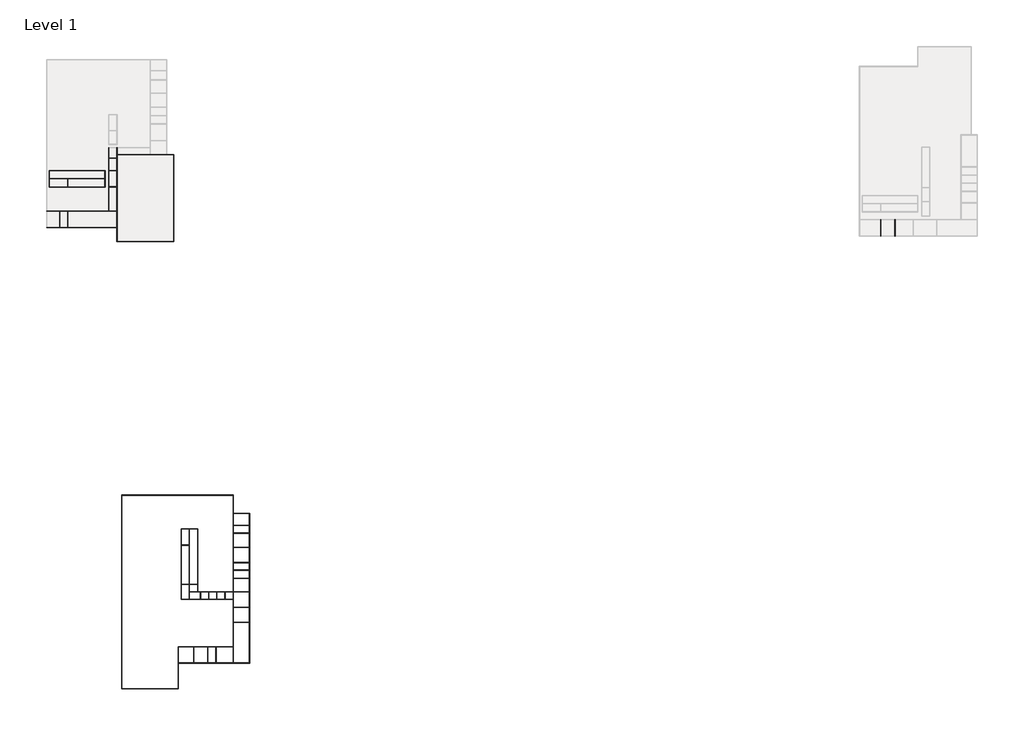
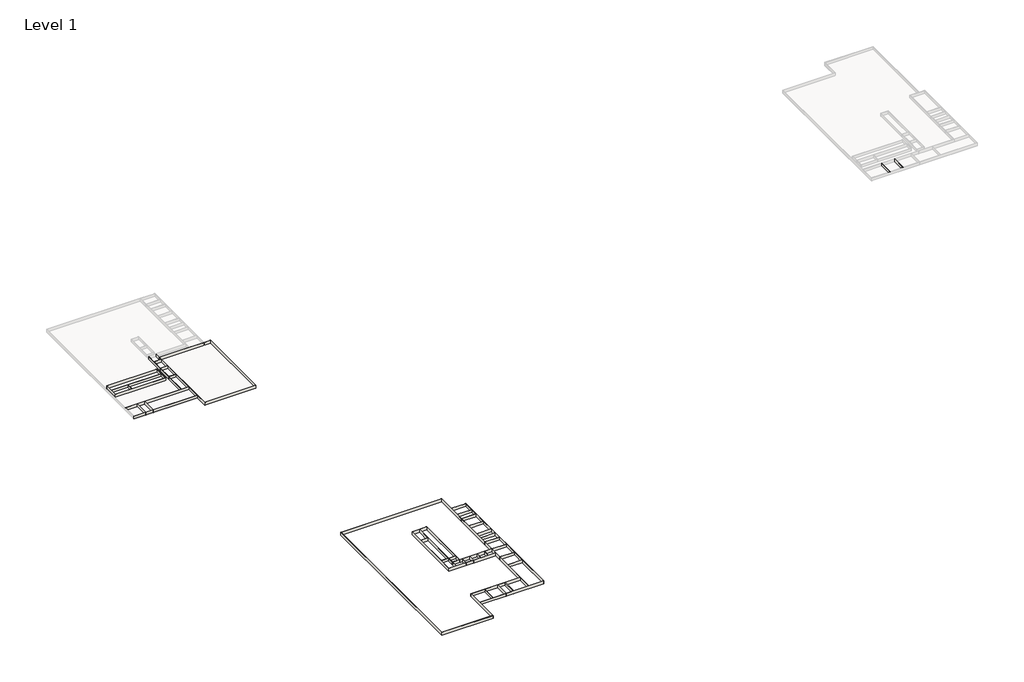
# One storey, part 1 of 4: 54 walls.
# Revit data of these elements (continued)
# Room at (-155472.417, -565316.915) mm, phase "New Construction", upper level "Level 1", upper offset 10' - 0", lower offset 0' - 0"
#   Number = "190"
#   Name = "SPORTING GOODS"
# Room at (-138960.745, -565316.915) mm, phase "New Construction", upper level "Level 1", upper offset 10' - 0", lower offset 0' - 0"
#   Number = "191"
#   Name = "SUBWAY"
# Room at (-127746.861, -565316.915) mm, phase "New Construction", upper level "Level 1", upper offset 10' - 0", lower offset 0' - 0"
#   Number = "192"
#   Name = "LOCKER ROOMS"
# Room at (-108757.336, -565316.915) mm, phase "New Construction", upper level "Level 1", upper offset 10' - 0", lower offset 0' - 0"
#   Number = "193"
#   Name = "AEROBICS/YOGA"
# Room at (-93779.435, -521588.2) mm, phase "New Construction", upper level "Level 1", upper offset 10' - 0", lower offset 0' - 0"
#   Number = "194"
#   Name = "KITCHEN/CONCESSIONS"
# Room at (-93779.435, -504532.187) mm, phase "New Construction", upper level "Level 1", upper offset 10' - 0", lower offset 0' - 0"
#   Number = "195"
#   Name = "ENTRY/RECEPTION"
# Room at (-93779.435, -487084.233) mm, phase "New Construction", upper level "Level 1", upper offset 10' - 0", lower offset 0' - 0"
#   Number = "196"
#   Name = "CLASSROOM"
# Room at (-93555.18, -477128.088) mm, phase "New Construction", upper level "Level 1", upper offset 10' - 0", lower offset 0' - 0"
#   Number = "197"
#   Name = "LOCKER ROOM"
# Room at (-93779.435, -454815.723) mm, phase "New Construction", upper level "Level 1", upper offset 10' - 0", lower offset 0' - 0"
#   Number = "198"
#   Name = "CLASSROOM"
# Room at (-93779.435, -436939.158) mm, phase "New Construction", upper level "Level 1", upper offset 10' - 0", lower offset 0' - 0"
#   Number = "199"
#   Name = "CLASSROOM"
# Room at (-93779.435, -416167.524) mm, phase "New Construction", upper level "Level 1", upper offset 10' - 0", lower offset 0' - 0"
#   Number = "200"
#   Name = "STORAGE"
# Room at (-147206.69, -458248.169) mm, phase "New Construction", upper level "Level 1", upper offset 10' - 0", lower offset 0' - 0"
#   Number = "201"
#   Name = "THE ALLEY"
# Room at (-156348.333, -470420.161) mm, phase "New Construction", upper level "Level 1", upper offset 10' - 0", lower offset 0' - 0"
#   Number = "202"
#   Name = "FITNESS"
# Room at (-156348.333, -434312.218) mm, phase "New Construction", upper level "Level 1", upper offset 10' - 0", lower offset 0' - 0"
#   Number = "203"
#   Name = "STOR. / MECH."
# Room at (-134717.782, -499647.502) mm, phase "New Construction", upper level "Level 1", upper offset 10' - 0", lower offset 0' - 0"
#   Number = "204"
#   Name = "CLASSR."
# Room at (-125440.864, -499647.502) mm, phase "New Construction", upper level "Level 1", upper offset 10' - 0", lower offset 0' - 0"
#   Number = "205"
#   Name = "CLASSR."
# Room at (-115822.884, -499647.502) mm, phase "New Construction", upper level "Level 1", upper offset 10' - 0", lower offset 0' - 0"
#   Number = "206"
#   Name = "CLASSR."
# Room at (-107978.431, -499647.502) mm, phase "New Construction", upper level "Level 1", upper offset 10' - 0", lower offset 0' - 0"
#   Number = "207"
#   Name = "CLASSR."
# Room at (-145836.44, -499647.502) mm, phase "New Construction", upper level "Level 1", upper offset 10' - 0", lower offset 0' - 0"
#   Number = "208"
#   Name = "CLASSROOM"
# Room at (-146992.866, -491393.774) mm, phase "New Construction", upper level "Level 1", upper offset 10' - 0", lower offset 0' - 0"
#   Number = "209"
#   Name = "CLASSR."
# Room at (-155983.587, -494826.219) mm, phase "New Construction", upper level "Level 1", upper offset 10' - 0", lower offset 0' - 0"
#   Number = "210"
#   Name = "CLASSROOM"
# Room at (-93779.435, -425215.001) mm, phase "New Construction", upper level "Level 1", upper offset 10' - 0", lower offset 0' - 0"
#   Number = "211"
#   Name = "CONFERENCE"
# Room at (-93779.435, -467011.221) mm, phase "New Construction", upper level "Level 1", upper offset 10' - 0", lower offset 0' - 0"
#   Number = "212"
#   Name = "LOCKER ROOM"
# Room at (672322.647, -64446.408) mm, phase "New Construction", upper level "Level 1", upper offset 10' - 0", lower offset 0' - 0"
#   Number = "91"
#   Name = "CLASSROOM"
# Room, not placed, phase "New Construction", upper offset 0' - 0", lower offset 0' - 0"
#   Number = "92"
#   Name = "CLASSROOM"
# Room, not placed, phase "New Construction", upper offset 0' - 0", lower offset 0' - 0"
#   Number = "2"
#   Name = "Room"
# Room, not placed, phase "New Construction", upper offset 0' - 0", lower offset 0' - 0"
#   Number = "5"
#   Name = "Room"
# Room, not placed, phase "New Construction", upper offset 0' - 0", lower offset 0' - 0"
#   Number = "8"
#   Name = "Room"
# Room, not placed, phase "New Construction", upper offset 0' - 0", lower offset 0' - 0"
#   Number = "9"
#   Name = "Room"
# Room, not placed, phase "New Construction", upper offset 0' - 0", lower offset 0' - 0"
#   Number = "10"
#   Name = "Clinic"
# Room, not placed, phase "New Construction", upper offset 0' - 0", lower offset 0' - 0"
#   Number = "14"
#   Name = "Room"
# Room, not placed, phase "New Construction", upper offset 0' - 0", lower offset 0' - 0"
#   Number = "15"
#   Name = "Room"
# Room, not placed, phase "New Construction", upper offset 0' - 0", lower offset 0' - 0"
#   Number = "16"
#   Name = "Room"
# Room, not placed, phase "New Construction", upper offset 0' - 0", lower offset 0' - 0"
#   Number = "17"
#   Name = "Room"
# Room, not placed, phase "New Construction", upper offset 0' - 0", lower offset 0' - 0"
#   Number = "18"
#   Name = "Room"
# Room, not placed, phase "New Construction", upper offset 0' - 0", lower offset 0' - 0"
#   Number = "19"
#   Name = "Room"
# Room, not placed, phase "New Construction", upper offset 0' - 0", lower offset 0' - 0"
#   Number = "21"
#   Name = "Room"
# Room, not placed, phase "New Construction", upper offset 0' - 0", lower offset 0' - 0"
#   Number = "22"
#   Name = "Room"
# Room, not placed, phase "New Construction", upper offset 0' - 0", lower offset 0' - 0"
#   Number = "23"
#   Name = "Room"
# Room, not placed, phase "New Construction", upper offset 0' - 0", lower offset 0' - 0"
#   Number = "24"
#   Name = "Room"
# Room, not placed, phase "New Construction", upper offset 0' - 0", lower offset 0' - 0"
#   Number = "25"
#   Name = "Room"
# Room, not placed, phase "New Construction", upper offset 0' - 0", lower offset 0' - 0"
#   Number = "29"
#   Name = "Room"
# Room, not placed, phase "New Construction", upper offset 0' - 0", lower offset 0' - 0"
#   Number = "32"
#   Name = "Room"
# Room at (670326.663, -55930.702) mm, phase "New Construction", upper level "Level 1", upper offset 10' - 0", lower offset 0' - 0"
#   Number = "96"
#   Name = "CLASSROOM"
# Room at (-192435.228, 94765.263) mm, phase "New Construction", upper level "Level 1", upper offset 10' - 0", lower offset 0' - 0"
#   Number = "117"
#   Name = "Storage/Mech"
# Room at (-192065.488, 78761.477) mm, phase "New Construction", upper level "Level 1", upper offset 10' - 0", lower offset 0' - 0"
#   Number = "118"
#   Name = "OFFICES/CONF."
# Room at (-180671.025, 34032.43) mm, phase "New Construction", upper level "Level 1", upper offset 10' - 0", lower offset 0' - 0"
#   Number = "119"
#   Name = "LOCKEROOM"
# Room at (-185204.588, 17190.064) mm, phase "New Construction", upper level "Level 1", upper offset 10' - 0", lower offset 0' - 0"
#   Number = "120"
#   Name = "KITCHEN/CONCESSIONS"
# Room at (-180671.025, 4452.403) mm, phase "New Construction", upper level "Level 1", upper offset 10' - 0", lower offset 0' - 0"
#   Number = "121"
#   Name = "ENTRY/RECEPTION"
# Room at (-253366.354, -79471.173) mm, phase "New Construction", upper level "Level 1", upper offset 10' - 0", lower offset 0' - 0"
#   Number = "122"
#   Name = "CLINIC"
# Room at (-237121.541, -52576.364) mm, phase "New Construction", upper level "Level 1", upper offset 10' - 0", lower offset 0' - 0"
#   Number = "123"
#   Name = "CLASSROOM"
# Room at (-237121.541, -37934.562) mm, phase "New Construction", upper level "Level 1", upper offset 10' - 0", lower offset 0' - 0"
#   Number = "124"
#   Name = "CLASSROOM"
# Room at (-237121.541, 33693.172) mm, phase "New Construction", upper level "Level 1", upper offset 10' - 0", lower offset 0' - 0"
#   Number = "125"
#   Name = "CLASSROOM/SPINNING"
# Room at (-292404.606, -82678.747) mm, phase "New Construction", upper level "Level 1", upper offset 10' - 0", lower offset 0' - 0"
#   Number = "126"
#   Name = "SUBWAY"
# Room at (-307196.076, -82678.747) mm, phase "New Construction", upper level "Level 1", upper offset 10' - 0", lower offset 0' - 0"
#   Number = "127"
#   Name = "SPORTING GOODS"
# Room at (-251800.403, -38023.513) mm, phase "New Construction", upper level "Level 1", upper offset 10' - 0", lower offset 0' - 0"
#   Number = "128"
#   Name = "FITNESS"
# Room at (-294952.877, -38023.513) mm, phase "New Construction", upper level "Level 1", upper offset 10' - 0", lower offset 0' - 0"
#   Number = "129"
#   Name = "STOR./MECH."
# Room at (-282267.022, -30030.186) mm, phase "New Construction", upper level "Level 1", upper offset 10' - 0", lower offset 0' - 0"
#   Number = "130"
#   Name = "THE ALLEY"
# Room at (-237121.541, -4894.498) mm, phase "New Construction", upper level "Level 1", upper offset 10' - 0", lower offset 0' - 0"
#   Number = "136"
#   Name = "CLASSROOM"
# Room, not placed, phase "New Construction", upper offset 0' - 0", lower offset 0' - 0"
#   Number = "33"
#   Name = "Room"
# Room, not placed, phase "New Construction", upper offset 0' - 0", lower offset 0' - 0"
#   Number = "34"
#   Name = "Room"
# Room, not placed, phase "New Construction", upper offset 0' - 0", lower offset 0' - 0"
#   Number = "35"
#   Name = "Room"
# Room, not placed, phase "New Construction", upper offset 0' - 0", lower offset 0' - 0"
#   Number = "36"
#   Name = "Room"
# Room, not placed, phase "New Construction", upper offset 0' - 0", lower offset 0' - 0"
#   Number = "37"
#   Name = "Room"
# Room, not placed, phase "New Construction", upper offset 0' - 0", lower offset 0' - 0"
#   Number = "38"
#   Name = "Room"
# Room, not placed, phase "New Construction", upper offset 0' - 0", lower offset 0' - 0"
#   Number = "39"
#   Name = "Clinic"
# Room, not placed, phase "New Construction", upper offset 0' - 0", lower offset 0' - 0"
#   Number = "40"
#   Name = "Room"
# Room, not placed, phase "New Construction", upper offset 0' - 0", lower offset 0' - 0"
#   Number = "41"
#   Name = "Room"
# Room, not placed, phase "New Construction", upper offset 0' - 0", lower offset 0' - 0"
#   Number = "42"
#   Name = "Room"
# Room, not placed, phase "New Construction", upper offset 0' - 0", lower offset 0' - 0"
#   Number = "43"
#   Name = "Room"
# Room, not placed, phase "New Construction", upper offset 0' - 0", lower offset 0' - 0"
#   Number = "44"
#   Name = "Room"
# Room, not placed, phase "New Construction", upper offset 0' - 0", lower offset 0' - 0"
#   Number = "45"
#   Name = "Fitness"
# Room, not placed, phase "New Construction", upper offset 0' - 0", lower offset 0' - 0"
#   Number = "46"
#   Name = "Storage"
# Room, not placed, phase "New Construction", upper offset 0' - 0", lower offset 0' - 0"
#   Number = "47"
#   Name = "The Alley"
# Room at (-183206.314, 67966.133) mm, phase "New Construction", upper level "Level 1", upper offset 10' - 0", lower offset 0' - 0"
#   Number = "137"
#   Name = "Classroom"
# Room at (1588361.539, 84512.004) mm, phase "New Construction", upper level "Level 1", upper offset 10' - 0", lower offset 0' - 0"
#   Number = "90"
#   Name = "Room"
# Room at (2460506.754, -35163.043) mm, phase "New Construction", upper level "Level 1", upper offset 10' - 0", lower offset 0' - 0"
#   Number = "138"
#   Name = "CLINIC"
# Room at (2488320.402, -35163.043) mm, phase "New Construction", upper level "Level 1", upper offset 10' - 0", lower offset 0' - 0"
#   Number = "139"
#   Name = "KITCHEN/CONCESSIONS"
# Room at (2504050.059, -35163.043) mm, phase "New Construction", upper level "Level 1", upper offset 10' - 0", lower offset 0' - 0"
#   Number = "140"
#   Name = "XCEL ENTRANCE"
# Room at (2522624.517, -33639.043) mm, phase "New Construction", upper level "Level 1", upper offset 10' - 0", lower offset 0' - 0"
#   Number = "141"
#   Name = "LOCKER ROOM"
# Room at (2543990.806, -35163.043) mm, phase "New Construction", upper level "Level 1", upper offset 10' - 0", lower offset 0' - 0"
#   Number = "142"
#   Name = "RETAIL"
# Room at (2569660.809, -35163.043) mm, phase "New Construction", upper level "Level 1", upper offset 10' - 0", lower offset 0' - 0"
#   Number = "143"
#   Name = "RETAIL"
# Room at (2589948.392, -35163.043) mm, phase "New Construction", upper level "Level 1", upper offset 10' - 0", lower offset 0' - 0"
#   Number = "144"
#   Name = "RETAIL"
# Room at (2605324.829, -28341.246) mm, phase "New Construction", upper level "Level 1", upper offset 10' - 0", lower offset 0' - 0"
#   Number = "145"
#   Name = "RETAIL"
# Room at (2605324.829, -1636.162) mm, phase "New Construction", upper level "Level 1", upper offset 10' - 0", lower offset 0' - 0"
#   Number = "146"
#   Name = "RETAIL"
# Room at (2605324.829, 21963.679) mm, phase "New Construction", upper level "Level 1", upper offset 10' - 0", lower offset 0' - 0"
#   Number = "147"
#   Name = "RETAIL"
# Room at (2605324.829, 48047.714) mm, phase "New Construction", upper level "Level 1", upper offset 10' - 0", lower offset 0' - 0"
#   Number = "148"
#   Name = "RETAIL"
# Room at (2605324.829, 67248.226) mm, phase "New Construction", upper level "Level 1", upper offset 10' - 0", lower offset 0' - 0"
#   Number = "149"
#   Name = "RETAIL"
# Room at (2522593.022, -35170.673) mm, phase "New Construction", upper level "Level 1", upper offset 10' - 0", lower offset 0' - 0"
#   Number = "150"
#   Name = "LOCKER ROOM"
